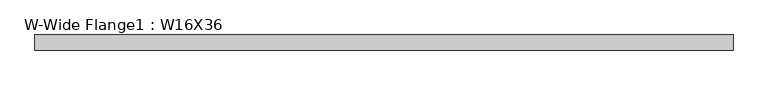
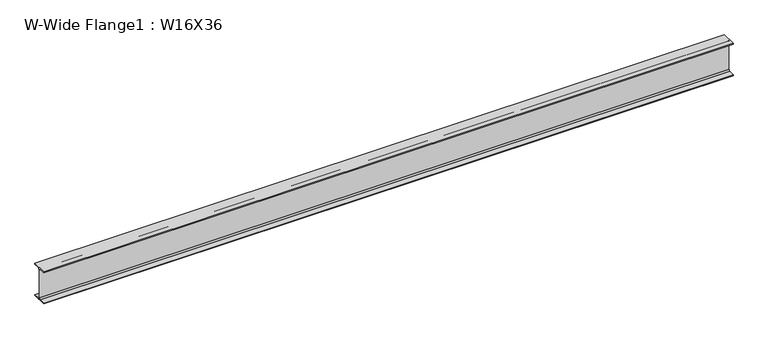
"""IFC4 building model written with IfcOpenShell, lengths in millimetres: beam geometry, W-Wide Flange1 : W16X36."""

from ifc_helpers import new_model, si_unit, point, frame, frame_2d, origin, place, context, project, spatial, polyline, circle_curve, trimmed, segment, composite_curve, outline, extrude, source, transform, mapped, element, save


def w_wide_flange1_w16x36_a1f35571(model_context):
    return source(origin(), model_context, "Body", "SweptSolid", [
        extrude(outline(composite_curve([segment(polyline([(88.773, -191.008), (88.773, -201.93), (-88.773, -201.93), (-88.773, -191.008), (-21.3995, -191.008)]), True, "CONTINUOUS"), segment(trimmed(circle_curve(frame_2d((-21.3995, -173.355)), 17.653), [point((-21.3995, -191.008))], [point((-3.7465, -173.355))], True, "CARTESIAN"), True, "CONTINUOUS"), segment(polyline([(-3.7465, -173.355), (-3.7465, 173.355)]), True, "CONTINUOUS"), segment(trimmed(circle_curve(frame_2d((-21.3995, 173.355)), 17.653), [point((-3.7465, 173.355))], [point((-21.3995, 191.008))], True, "CARTESIAN"), True, "CONTINUOUS"), segment(polyline([(-21.3995, 191.008), (-88.773, 191.008), (-88.773, 201.93), (88.773, 201.93), (88.773, 191.008), (21.3995, 191.008)]), True, "CONTINUOUS"), segment(trimmed(circle_curve(frame_2d((21.3995, 173.355)), 17.653), [point((21.3995, 191.008))], [point((3.7465, 173.355))], True, "CARTESIAN"), True, "CONTINUOUS"), segment(polyline([(3.7465, 173.355), (3.7465, -173.355)]), True, "CONTINUOUS"), segment(trimmed(circle_curve(frame_2d((21.3995, -173.355)), 17.653), [point((3.7465, -173.355))], [point((21.3995, -191.008))], True, "CARTESIAN"), True, "CONTINUOUS"), segment(polyline([(21.3995, -191.008), (88.773, -191.008)]), True, "CONTINUOUS")], self_intersect=False)), frame((-4053.15, 0.0, 0.0), z_axis=(1.0, 0.0, 0.0), x_axis=(0.0, 1.0, 0.0)), (0.0, 0.0, 1.0), 8197.7056202),
    ])


if __name__ == "__main__":
    model = new_model("IFC4")
    model_context = context("Model", 3, world=origin())
    ifc_project = project(units=[si_unit("LENGTHUNIT", "METRE", prefix="MILLI")], contexts=[model_context])
    site = spatial("IfcSite", under=ifc_project)
    building = spatial("IfcBuilding", under=site)
    placement = place(None, origin())
    w_wide_flange1_w16x36_shape = w_wide_flange1_w16x36_a1f35571(model_context)
    element("IfcBeam", 1, ObjectType="W-Wide Flange1 : W16X36", at=placement, inside=building, context=model_context, shape_type="MappedRepresentation", body=[
        mapped(w_wide_flange1_w16x36_shape, transform((0.0, 0.0, 0.0), x_axis=(1.0, 0.0, 0.0), y_axis=(0.0, 1.0, 0.0), z_axis=(0.0, 0.0, 1.0))),
    ])
    save(model, "model.ifc")

# Revit data of these elements
# Type "W-Wide Flange1 : W16X36"
#   Assembly Code = "B10"
#   W = 36
#   Start Extension Calculation [instance default] = 10' - 0"
#   Start Extension [instance default] = -0' - 0 1/2"
#   End Extension Calculation [instance default] = 10' - 0"
#   End Extension [instance default] = -0' - 0 1/2"
#   Length [instance default] = 5' - 0"
#   bf = 0' - 6.99"
#   d = 1' - 3.9"
#   k = 0' - 1 1/8"
#   k2 = 0' - 0.695"
#   tf = 0' - 0.43"
#   tw = 0' - 0.295"
#   A = 0.0736111 SF
#   Structural Material [instance default] = Metal - Steel - ASTM A992
# Element 1 (IfcBeam, "W-Wide Flange1 : W16X36")
#   Materials on its faces: "Metal - Steel - ASTM A992"
# Materials
#   "Metal - Steel - ASTM A992": class "Metal", colour RGB 199 199 199, transparency 0
